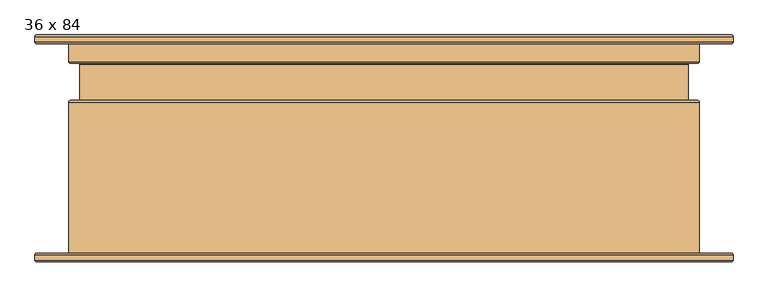
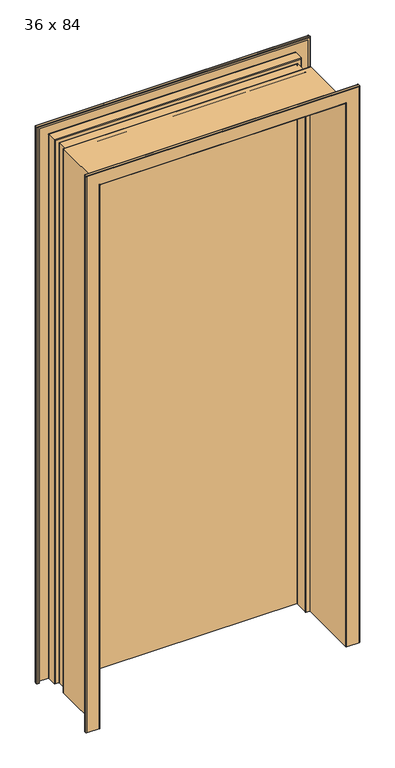
"""IFC4 building model written with IfcOpenShell, lengths in millimetres: door geometry, Door-Dunbarton_Doors-Hollow_Metal_Core : 36 x 84."""

from ifc_helpers import new_model, si_unit, frame, origin, origin_with_axes, place, context, project, spatial, polyline, circle_curve, ellipse_curve, outline, extrude, source, transform, mapped, element, save
from ifc_brep_helpers import plane_surface, cylinder_surface, revolved_surface, advanced_brep


def door_36_x_84_73b2aa22(model_context):
    return source(origin(), model_context, "Body", "SolidModel", [
        advanced_brep(
        [(-505.42825, -152.4635, 0.0), (-500.0625, -152.4635, 0.0), (-500.0625, -154.01925, 0.0), (-505.42825, -154.01925, 0.0), (-506.44425, -155.03525, 0.0), (-506.44425, -162.56, 0.0), (-505.42825, -163.576, 0.0), (-459.77175, -163.576, 0.0), (-458.75575, -162.56, 0.0), (-458.75575, 67.21475, 0.0), (-456.184, 69.7865, 0.0), (-443.89675, 69.7865, 0.0), (-442.88075, 70.8025, 0.0), (-442.88075, 122.5931, 0.0), (-443.89675, 123.6091, 0.0), (-456.184, 123.6091, 0.0), (-458.75575, 126.18085, 0.0), (-458.75575, 162.4965, 0.0), (-459.77175, 163.5125, 0.0), (-505.42825, 163.5125, 0.0), (-506.44425, 162.4965, 0.0), (-506.44425, 154.97175, 0.0), (-505.42825, 153.95575, 0.0), (-500.0625, 153.95575, 0.0), (-500.0625, 152.4, 0.0), (-505.42825, 152.4, 0.0), (-508.0, 154.97175, 0.0), (-508.0, 162.4965, 0.0), (-505.42825, 165.06825, 0.0), (-459.77175, 165.06825, 0.0), (-457.2, 162.4965, 0.0), (-457.2, 126.18085, 0.0), (-456.184, 125.16485, 0.0), (-443.89675, 125.16485, 0.0), (-441.325, 122.5931, 0.0), (-441.325, 70.8025, 0.0), (-443.89675, 68.23075, 0.0), (-456.184, 68.23075, 0.0), (-457.2, 67.21475, 0.0), (-457.2, -162.56, 0.0), (-459.77175, -165.13175, 0.0), (-505.42825, -165.13175, 0.0), (-508.0, -162.56, 0.0), (-508.0, -155.03525, 0.0), (-508.0, -155.03525, 2184.4), (-505.42825, -152.4635, 2181.82825), (-508.0, -162.56, 2184.4), (-505.42825, -165.13175, 2181.82825), (-459.77175, -165.13175, 2136.17175), (459.77175, -165.13175, 2136.17175), (459.77175, -165.13175, 0.0), (505.42825, -165.13175, 0.0), (505.42825, -165.13175, 2181.82825), (-457.2, -162.56, 2133.6), (-457.2, 67.21475, 2133.6), (-456.184, 68.23075, 2132.584), (-443.89675, 68.23075, 2120.29675), (443.89675, 68.23075, 2120.29675), (443.89675, 68.23075, 0.0), (456.184, 68.23075, 0.0), (456.184, 68.23075, 2132.584), (-441.325, 70.8025, 2117.725), (-441.325, 122.5931, 2117.725), (-443.89675, 125.16485, 2120.29675), (-456.184, 125.16485, 2132.584), (456.184, 125.16485, 2132.584), (456.184, 125.16485, 0.0), (443.89675, 125.16485, 0.0), (443.89675, 125.16485, 2120.29675), (-457.2, 126.18085, 2133.6), (-457.2, 162.4965, 2133.6), (-459.77175, 165.06825, 2136.17175), (-505.42825, 165.06825, 2181.82825), (505.42825, 165.06825, 2181.82825), (505.42825, 165.06825, 0.0), (459.77175, 165.06825, 0.0), (459.77175, 165.06825, 2136.17175), (-508.0, 162.4965, 2184.4), (-508.0, 154.97175, 2184.4), (-505.42825, 152.4, 2181.82825), (-500.0625, 152.4, 2176.4625), (500.0625, 152.4, 2176.4625), (500.0625, 152.4, 0.0), (505.42825, 152.4, 0.0), (505.42825, 152.4, 2181.82825), (-500.0625, 153.95575, 2176.4625), (-505.42825, 153.95575, 2181.82825), (505.42825, 153.95575, 2181.82825), (505.42825, 153.95575, 0.0), (500.0625, 153.95575, 0.0), (500.0625, 153.95575, 2176.4625), (-506.44425, 154.97175, 2182.84425), (-506.44425, 162.4965, 2182.84425), (-505.42825, 163.5125, 2181.82825), (-459.77175, 163.5125, 2136.17175), (459.77175, 163.5125, 2136.17175), (459.77175, 163.5125, 0.0), (505.42825, 163.5125, 0.0), (505.42825, 163.5125, 2181.82825), (-458.75575, 162.4965, 2135.15575), (-458.75575, 126.18085, 2135.15575), (-456.184, 123.6091, 2132.584), (-443.89675, 123.6091, 2120.29675), (443.89675, 123.6091, 2120.29675), (443.89675, 123.6091, 0.0), (456.184, 123.6091, 0.0), (456.184, 123.6091, 2132.584), (-442.88075, 122.5931, 2119.28075), (-442.88075, 70.8025, 2119.28075), (-443.89675, 69.7865, 2120.29675), (-456.184, 69.7865, 2132.584), (456.184, 69.7865, 2132.584), (456.184, 69.7865, 0.0), (443.89675, 69.7865, 0.0), (443.89675, 69.7865, 2120.29675), (-458.75575, 67.21475, 2135.15575), (-458.75575, -162.56, 2135.15575), (-459.77175, -163.576, 2136.17175), (-505.42825, -163.576, 2181.82825), (505.42825, -163.576, 2181.82825), (505.42825, -163.576, 0.0), (459.77175, -163.576, 0.0), (459.77175, -163.576, 2136.17175), (-506.44425, -162.56, 2182.84425), (-506.44425, -155.03525, 2182.84425), (-505.42825, -154.01925, 2181.82825), (-500.0625, -154.01925, 2176.4625), (500.0625, -154.01925, 2176.4625), (500.0625, -154.01925, 0.0), (505.42825, -154.01925, 0.0), (505.42825, -154.01925, 2181.82825), (-500.0625, -152.4635, 2176.4625), (505.42825, -152.4635, 2181.82825), (505.42825, -152.4635, 0.0), (500.0625, -152.4635, 0.0), (500.0625, -152.4635, 2176.4625), (508.0, -155.03525, 2184.4), (508.0, -162.56, 2184.4), (457.2, -162.56, 2133.6), (457.2, 67.21475, 2133.6), (441.325, 70.8025, 2117.725), (441.325, 122.5931, 2117.725), (457.2, 126.18085, 2133.6), (457.2, 162.4965, 2133.6), (508.0, 162.4965, 2184.4), (508.0, 154.97175, 2184.4), (506.44425, 154.97175, 2182.84425), (506.44425, 162.4965, 2182.84425), (458.75575, 162.4965, 2135.15575), (458.75575, 126.18085, 2135.15575), (442.88075, 122.5931, 2119.28075), (442.88075, 70.8025, 2119.28075), (458.75575, 67.21475, 2135.15575), (458.75575, -162.56, 2135.15575), (506.44425, -162.56, 2182.84425), (506.44425, -155.03525, 2182.84425), (508.0, -155.03525, 0.0), (508.0, -162.56, 0.0), (457.2, -162.56, 0.0), (457.2, 67.21475, 0.0), (441.325, 70.8025, 0.0), (441.325, 122.5931, 0.0), (457.2, 126.18085, 0.0), (457.2, 162.4965, 0.0), (508.0, 162.4965, 0.0), (508.0, 154.97175, 0.0), (506.44425, 154.97175, 0.0), (506.44425, 162.4965, 0.0), (458.75575, 162.4965, 0.0), (458.75575, 126.18085, 0.0), (442.88075, 122.5931, 0.0), (442.88075, 70.8025, 0.0), (458.75575, 67.21475, 0.0), (458.75575, -162.56, 0.0), (506.44425, -162.56, 0.0), (506.44425, -155.03525, 0.0)],
        [
            (0, 1),
            (1, 2),
            (2, 3),
            (3, 4, circle_curve(frame((-505.42825, -155.03525, 0.0), z_axis=(0.0, 0.0, 1.0), x_axis=(0.0, 1.0, 0.0)), 1.016)),
            (4, 5),
            (5, 6, circle_curve(frame((-505.42825, -162.56, 0.0), z_axis=(0.0, 0.0, 1.0), x_axis=(0.0, 1.0, 0.0)), 1.016)),
            (6, 7),
            (7, 8, circle_curve(frame((-459.77175, -162.56, 0.0), z_axis=(0.0, 0.0, 1.0), x_axis=(0.0, 1.0, 0.0)), 1.016)),
            (8, 9),
            (9, 10, circle_curve(frame((-456.184, 67.21475, 0.0), z_axis=(0.0, 0.0, -1.0), x_axis=(0.0, 1.0, 0.0)), 2.57175)),
            (10, 11),
            (11, 12, circle_curve(frame((-443.89675, 70.8025, 0.0), z_axis=(0.0, 0.0, 1.0), x_axis=(0.0, 1.0, 0.0)), 1.016)),
            (12, 13),
            (13, 14, circle_curve(frame((-443.89675, 122.5931, 0.0), z_axis=(0.0, 0.0, 1.0), x_axis=(0.0, 1.0, 0.0)), 1.016)),
            (14, 15),
            (15, 16, circle_curve(frame((-456.184, 126.18085, 0.0), z_axis=(0.0, 0.0, -1.0), x_axis=(0.0, 1.0, 0.0)), 2.57175)),
            (16, 17),
            (17, 18, circle_curve(frame((-459.77175, 162.4965, 0.0), z_axis=(0.0, 0.0, 1.0), x_axis=(0.0, 1.0, 0.0)), 1.016)),
            (18, 19),
            (19, 20, circle_curve(frame((-505.42825, 162.4965, 0.0), z_axis=(0.0, 0.0, 1.0), x_axis=(0.0, 1.0, 0.0)), 1.016)),
            (20, 21),
            (21, 22, circle_curve(frame((-505.42825, 154.97175, 0.0), z_axis=(0.0, 0.0, 1.0), x_axis=(0.0, 1.0, 0.0)), 1.016)),
            (22, 23),
            (23, 24),
            (24, 25),
            (25, 26, circle_curve(frame((-505.42825, 154.97175, 0.0), z_axis=(0.0, 0.0, -1.0), x_axis=(0.0, 1.0, 0.0)), 2.57175)),
            (26, 27),
            (27, 28, circle_curve(frame((-505.42825, 162.4965, 0.0), z_axis=(0.0, 0.0, -1.0), x_axis=(0.0, 1.0, 0.0)), 2.57175)),
            (28, 29),
            (29, 30, circle_curve(frame((-459.77175, 162.4965, 0.0), z_axis=(0.0, 0.0, -1.0), x_axis=(0.0, 1.0, 0.0)), 2.57175)),
            (30, 31),
            (31, 32, circle_curve(frame((-456.184, 126.18085, 0.0), z_axis=(0.0, 0.0, 1.0), x_axis=(0.0, 1.0, 0.0)), 1.016)),
            (32, 33),
            (33, 34, circle_curve(frame((-443.89675, 122.5931, 0.0), z_axis=(0.0, 0.0, -1.0), x_axis=(0.0, 1.0, 0.0)), 2.57175)),
            (34, 35),
            (35, 36, circle_curve(frame((-443.89675, 70.8025, 0.0), z_axis=(0.0, 0.0, -1.0), x_axis=(0.0, 1.0, 0.0)), 2.57175)),
            (36, 37),
            (37, 38, circle_curve(frame((-456.184, 67.21475, 0.0), z_axis=(0.0, 0.0, 1.0), x_axis=(0.0, 1.0, 0.0)), 1.016)),
            (38, 39),
            (39, 40, circle_curve(frame((-459.77175, -162.56, 0.0), z_axis=(0.0, 0.0, -1.0), x_axis=(0.0, 1.0, 0.0)), 2.57175)),
            (40, 41),
            (41, 42, circle_curve(frame((-505.42825, -162.56, 0.0), z_axis=(0.0, 0.0, -1.0), x_axis=(0.0, 1.0, 0.0)), 2.57175)),
            (42, 43),
            (43, 0, circle_curve(frame((-505.42825, -155.03525, 0.0), z_axis=(0.0, 0.0, -1.0), x_axis=(0.0, 1.0, 0.0)), 2.57175)),
            (43, 44),
            (44, 45, ellipse_curve(frame((-505.42825, -155.03525, 2181.82825), z_axis=(-0.7071067811865475, 0.0, -0.7071067811865475), x_axis=(0.7071067811865474, 0.0, -0.7071067811865476)), 3.6370037, 2.57175)),
            (45, 0),
            (42, 46),
            (46, 44),
            (41, 47),
            (47, 46, ellipse_curve(frame((-505.42825, -162.56, 2181.82825), z_axis=(-0.7071067811865475, 0.0, -0.7071067811865475), x_axis=(0.7071067811865474, 0.0, -0.7071067811865476)), 3.6370037, 2.57175)),
            (40, 48),
            (48, 49),
            (49, 50),
            (50, 51),
            (51, 52),
            (52, 47),
            (39, 53),
            (53, 48, ellipse_curve(frame((-459.77175, -162.56, 2136.17175), z_axis=(-0.7071067811865475, 0.0, -0.7071067811865475), x_axis=(0.7071067811865474, 0.0, -0.7071067811865476)), 3.6370037, 2.57175)),
            (38, 54),
            (54, 53),
            (37, 55),
            (55, 54, ellipse_curve(frame((-456.184, 67.21475, 2132.584), z_axis=(0.7071067811865475, 0.0, 0.7071067811865475), x_axis=(-0.7071067811865474, 0.0, 0.7071067811865476)), 1.436841, 1.016)),
            (36, 56),
            (56, 57),
            (57, 58),
            (58, 59),
            (59, 60),
            (60, 55),
            (35, 61),
            (61, 56, ellipse_curve(frame((-443.89675, 70.8025, 2120.29675), z_axis=(-0.7071067811865475, 0.0, -0.7071067811865475), x_axis=(0.7071067811865474, 0.0, -0.7071067811865476)), 3.6370037, 2.57175)),
            (34, 62),
            (62, 61),
            (33, 63),
            (63, 62, ellipse_curve(frame((-443.89675, 122.5931, 2120.29675), z_axis=(-0.7071067811865475, 0.0, -0.7071067811865475), x_axis=(0.7071067811865474, 0.0, -0.7071067811865476)), 3.6370037, 2.57175)),
            (32, 64),
            (64, 65),
            (65, 66),
            (66, 67),
            (67, 68),
            (68, 63),
            (31, 69),
            (69, 64, ellipse_curve(frame((-456.184, 126.18085, 2132.584), z_axis=(0.7071067811865475, 0.0, 0.7071067811865475), x_axis=(-0.7071067811865474, 0.0, 0.7071067811865476)), 1.436841, 1.016)),
            (30, 70),
            (70, 69),
            (29, 71),
            (71, 70, ellipse_curve(frame((-459.77175, 162.4965, 2136.17175), z_axis=(-0.7071067811865475, 0.0, -0.7071067811865475), x_axis=(0.7071067811865474, 0.0, -0.7071067811865476)), 3.6370037, 2.57175)),
            (28, 72),
            (72, 73),
            (73, 74),
            (74, 75),
            (75, 76),
            (76, 71),
            (27, 77),
            (77, 72, ellipse_curve(frame((-505.42825, 162.4965, 2181.82825), z_axis=(-0.7071067811865475, 0.0, -0.7071067811865475), x_axis=(0.7071067811865474, 0.0, -0.7071067811865476)), 3.6370037, 2.57175)),
            (26, 78),
            (78, 77),
            (25, 79),
            (79, 78, ellipse_curve(frame((-505.42825, 154.97175, 2181.82825), z_axis=(-0.7071067811865475, 0.0, -0.7071067811865475), x_axis=(0.7071067811865474, 0.0, -0.7071067811865476)), 3.6370037, 2.57175)),
            (24, 80),
            (80, 81),
            (81, 82),
            (82, 83),
            (83, 84),
            (84, 79),
            (23, 85),
            (85, 80),
            (22, 86),
            (86, 87),
            (87, 88),
            (88, 89),
            (89, 90),
            (90, 85),
            (21, 91),
            (91, 86, ellipse_curve(frame((-505.42825, 154.97175, 2181.82825), z_axis=(0.7071067811865475, 0.0, 0.7071067811865475), x_axis=(-0.7071067811865474, 0.0, 0.7071067811865476)), 1.436841, 1.016)),
            (20, 92),
            (92, 91),
            (19, 93),
            (93, 92, ellipse_curve(frame((-505.42825, 162.4965, 2181.82825), z_axis=(0.7071067811865475, 0.0, 0.7071067811865475), x_axis=(-0.7071067811865474, 0.0, 0.7071067811865476)), 1.436841, 1.016)),
            (18, 94),
            (94, 95),
            (95, 96),
            (96, 97),
            (97, 98),
            (98, 93),
            (17, 99),
            (99, 94, ellipse_curve(frame((-459.77175, 162.4965, 2136.17175), z_axis=(0.7071067811865475, 0.0, 0.7071067811865475), x_axis=(-0.7071067811865474, 0.0, 0.7071067811865476)), 1.436841, 1.016)),
            (16, 100),
            (100, 99),
            (15, 101),
            (101, 100, ellipse_curve(frame((-456.184, 126.18085, 2132.584), z_axis=(-0.7071067811865475, 0.0, -0.7071067811865475), x_axis=(0.7071067811865474, 0.0, -0.7071067811865476)), 3.6370037, 2.57175)),
            (14, 102),
            (102, 103),
            (103, 104),
            (104, 105),
            (105, 106),
            (106, 101),
            (13, 107),
            (107, 102, ellipse_curve(frame((-443.89675, 122.5931, 2120.29675), z_axis=(0.7071067811865475, 0.0, 0.7071067811865475), x_axis=(-0.7071067811865474, 0.0, 0.7071067811865476)), 1.436841, 1.016)),
            (12, 108),
            (108, 107),
            (11, 109),
            (109, 108, ellipse_curve(frame((-443.89675, 70.8025, 2120.29675), z_axis=(0.7071067811865475, 0.0, 0.7071067811865475), x_axis=(-0.7071067811865474, 0.0, 0.7071067811865476)), 1.436841, 1.016)),
            (10, 110),
            (110, 111),
            (111, 112),
            (112, 113),
            (113, 114),
            (114, 109),
            (9, 115),
            (115, 110, ellipse_curve(frame((-456.184, 67.21475, 2132.584), z_axis=(-0.7071067811865475, 0.0, -0.7071067811865475), x_axis=(0.7071067811865474, 0.0, -0.7071067811865476)), 3.6370037, 2.57175)),
            (8, 116),
            (116, 115),
            (7, 117),
            (117, 116, ellipse_curve(frame((-459.77175, -162.56, 2136.17175), z_axis=(0.7071067811865475, 0.0, 0.7071067811865475), x_axis=(-0.7071067811865474, 0.0, 0.7071067811865476)), 1.436841, 1.016)),
            (6, 118),
            (118, 119),
            (119, 120),
            (120, 121),
            (121, 122),
            (122, 117),
            (5, 123),
            (123, 118, ellipse_curve(frame((-505.42825, -162.56, 2181.82825), z_axis=(0.7071067811865475, 0.0, 0.7071067811865475), x_axis=(-0.7071067811865474, 0.0, 0.7071067811865476)), 1.436841, 1.016)),
            (4, 124),
            (124, 123),
            (3, 125),
            (125, 124, ellipse_curve(frame((-505.42825, -155.03525, 2181.82825), z_axis=(0.7071067811865475, 0.0, 0.7071067811865475), x_axis=(-0.7071067811865474, 0.0, 0.7071067811865476)), 1.436841, 1.016)),
            (2, 126),
            (126, 127),
            (127, 128),
            (128, 129),
            (129, 130),
            (130, 125),
            (1, 131),
            (131, 126),
            (45, 132),
            (132, 133),
            (133, 134),
            (134, 135),
            (135, 131),
            (44, 136),
            (136, 132, ellipse_curve(frame((505.42825, -155.03525, 2181.82825), z_axis=(-0.7071067811865475, 0.0, 0.7071067811865475), x_axis=(-0.7071067811865476, 0.0, -0.7071067811865474)), 3.6370037, 2.57175)),
            (46, 137),
            (137, 136),
            (52, 137, ellipse_curve(frame((505.42825, -162.56, 2181.82825), z_axis=(-0.7071067811865475, 0.0, 0.7071067811865475), x_axis=(-0.7071067811865476, 0.0, -0.7071067811865474)), 3.6370037, 2.57175)),
            (53, 138),
            (138, 49, ellipse_curve(frame((459.77175, -162.56, 2136.17175), z_axis=(-0.7071067811865475, 0.0, 0.7071067811865475), x_axis=(-0.7071067811865476, 0.0, -0.7071067811865474)), 3.6370037, 2.57175)),
            (54, 139),
            (139, 138),
            (60, 139, ellipse_curve(frame((456.184, 67.21475, 2132.584), z_axis=(0.7071067811865475, 0.0, -0.7071067811865475), x_axis=(0.7071067811865476, 0.0, 0.7071067811865474)), 1.436841, 1.016)),
            (61, 140),
            (140, 57, ellipse_curve(frame((443.89675, 70.8025, 2120.29675), z_axis=(-0.7071067811865475, 0.0, 0.7071067811865475), x_axis=(-0.7071067811865476, 0.0, -0.7071067811865474)), 3.6370037, 2.57175)),
            (62, 141),
            (141, 140),
            (68, 141, ellipse_curve(frame((443.89675, 122.5931, 2120.29675), z_axis=(-0.7071067811865475, 0.0, 0.7071067811865475), x_axis=(-0.7071067811865476, 0.0, -0.7071067811865474)), 3.6370037, 2.57175)),
            (69, 142),
            (142, 65, ellipse_curve(frame((456.184, 126.18085, 2132.584), z_axis=(0.7071067811865475, 0.0, -0.7071067811865475), x_axis=(0.7071067811865476, 0.0, 0.7071067811865474)), 1.436841, 1.016)),
            (70, 143),
            (143, 142),
            (76, 143, ellipse_curve(frame((459.77175, 162.4965, 2136.17175), z_axis=(-0.7071067811865475, 0.0, 0.7071067811865475), x_axis=(-0.7071067811865476, 0.0, -0.7071067811865474)), 3.6370037, 2.57175)),
            (77, 144),
            (144, 73, ellipse_curve(frame((505.42825, 162.4965, 2181.82825), z_axis=(-0.7071067811865475, 0.0, 0.7071067811865475), x_axis=(-0.7071067811865476, 0.0, -0.7071067811865474)), 3.6370037, 2.57175)),
            (78, 145),
            (145, 144),
            (84, 145, ellipse_curve(frame((505.42825, 154.97175, 2181.82825), z_axis=(-0.7071067811865475, 0.0, 0.7071067811865475), x_axis=(-0.7071067811865476, 0.0, -0.7071067811865474)), 3.6370037, 2.57175)),
            (90, 81),
            (91, 146),
            (146, 87, ellipse_curve(frame((505.42825, 154.97175, 2181.82825), z_axis=(0.7071067811865475, 0.0, -0.7071067811865475), x_axis=(0.7071067811865476, 0.0, 0.7071067811865474)), 1.436841, 1.016)),
            (92, 147),
            (147, 146),
            (98, 147, ellipse_curve(frame((505.42825, 162.4965, 2181.82825), z_axis=(0.7071067811865475, 0.0, -0.7071067811865475), x_axis=(0.7071067811865476, 0.0, 0.7071067811865474)), 1.436841, 1.016)),
            (99, 148),
            (148, 95, ellipse_curve(frame((459.77175, 162.4965, 2136.17175), z_axis=(0.7071067811865475, 0.0, -0.7071067811865475), x_axis=(0.7071067811865476, 0.0, 0.7071067811865474)), 1.436841, 1.016)),
            (100, 149),
            (149, 148),
            (106, 149, ellipse_curve(frame((456.184, 126.18085, 2132.584), z_axis=(-0.7071067811865475, 0.0, 0.7071067811865475), x_axis=(-0.7071067811865476, 0.0, -0.7071067811865474)), 3.6370037, 2.57175)),
            (107, 150),
            (150, 103, ellipse_curve(frame((443.89675, 122.5931, 2120.29675), z_axis=(0.7071067811865475, 0.0, -0.7071067811865475), x_axis=(0.7071067811865476, 0.0, 0.7071067811865474)), 1.436841, 1.016)),
            (108, 151),
            (151, 150),
            (114, 151, ellipse_curve(frame((443.89675, 70.8025, 2120.29675), z_axis=(0.7071067811865475, 0.0, -0.7071067811865475), x_axis=(0.7071067811865476, 0.0, 0.7071067811865474)), 1.436841, 1.016)),
            (115, 152),
            (152, 111, ellipse_curve(frame((456.184, 67.21475, 2132.584), z_axis=(-0.7071067811865475, 0.0, 0.7071067811865475), x_axis=(-0.7071067811865476, 0.0, -0.7071067811865474)), 3.6370037, 2.57175)),
            (116, 153),
            (153, 152),
            (122, 153, ellipse_curve(frame((459.77175, -162.56, 2136.17175), z_axis=(0.7071067811865475, 0.0, -0.7071067811865475), x_axis=(0.7071067811865476, 0.0, 0.7071067811865474)), 1.436841, 1.016)),
            (123, 154),
            (154, 119, ellipse_curve(frame((505.42825, -162.56, 2181.82825), z_axis=(0.7071067811865475, 0.0, -0.7071067811865475), x_axis=(0.7071067811865476, 0.0, 0.7071067811865474)), 1.436841, 1.016)),
            (124, 155),
            (155, 154),
            (130, 155, ellipse_curve(frame((505.42825, -155.03525, 2181.82825), z_axis=(0.7071067811865475, 0.0, -0.7071067811865475), x_axis=(0.7071067811865476, 0.0, 0.7071067811865474)), 1.436841, 1.016)),
            (135, 127),
            (133, 156, circle_curve(frame((505.42825, -155.03525, 0.0), z_axis=(0.0, 0.0, -1.0), x_axis=(0.0, 1.0, 0.0)), 2.57175)),
            (156, 157),
            (157, 51, circle_curve(frame((505.42825, -162.56, 0.0), z_axis=(0.0, 0.0, -1.0), x_axis=(0.0, 1.0, 0.0)), 2.57175)),
            (50, 158, circle_curve(frame((459.77175, -162.56, 0.0), z_axis=(0.0, 0.0, -1.0), x_axis=(0.0, 1.0, 0.0)), 2.57175)),
            (158, 159),
            (159, 59, circle_curve(frame((456.184, 67.21475, 0.0), z_axis=(0.0, 0.0, 1.0), x_axis=(0.0, 1.0, 0.0)), 1.016)),
            (58, 160, circle_curve(frame((443.89675, 70.8025, 0.0), z_axis=(0.0, 0.0, -1.0), x_axis=(0.0, 1.0, 0.0)), 2.57175)),
            (160, 161),
            (161, 67, circle_curve(frame((443.89675, 122.5931, 0.0), z_axis=(0.0, 0.0, -1.0), x_axis=(0.0, 1.0, 0.0)), 2.57175)),
            (66, 162, circle_curve(frame((456.184, 126.18085, 0.0), z_axis=(0.0, 0.0, 1.0), x_axis=(0.0, 1.0, 0.0)), 1.016)),
            (162, 163),
            (163, 75, circle_curve(frame((459.77175, 162.4965, 0.0), z_axis=(0.0, 0.0, -1.0), x_axis=(0.0, 1.0, 0.0)), 2.57175)),
            (74, 164, circle_curve(frame((505.42825, 162.4965, 0.0), z_axis=(0.0, 0.0, -1.0), x_axis=(0.0, 1.0, 0.0)), 2.57175)),
            (164, 165),
            (165, 83, circle_curve(frame((505.42825, 154.97175, 0.0), z_axis=(0.0, 0.0, -1.0), x_axis=(0.0, 1.0, 0.0)), 2.57175)),
            (82, 89),
            (88, 166, circle_curve(frame((505.42825, 154.97175, 0.0), z_axis=(0.0, 0.0, 1.0), x_axis=(0.0, 1.0, 0.0)), 1.016)),
            (166, 167),
            (167, 97, circle_curve(frame((505.42825, 162.4965, 0.0), z_axis=(0.0, 0.0, 1.0), x_axis=(0.0, 1.0, 0.0)), 1.016)),
            (96, 168, circle_curve(frame((459.77175, 162.4965, 0.0), z_axis=(0.0, 0.0, 1.0), x_axis=(0.0, 1.0, 0.0)), 1.016)),
            (168, 169),
            (169, 105, circle_curve(frame((456.184, 126.18085, 0.0), z_axis=(0.0, 0.0, -1.0), x_axis=(0.0, 1.0, 0.0)), 2.57175)),
            (104, 170, circle_curve(frame((443.89675, 122.5931, 0.0), z_axis=(0.0, 0.0, 1.0), x_axis=(0.0, 1.0, 0.0)), 1.016)),
            (170, 171),
            (171, 113, circle_curve(frame((443.89675, 70.8025, 0.0), z_axis=(0.0, 0.0, 1.0), x_axis=(0.0, 1.0, 0.0)), 1.016)),
            (112, 172, circle_curve(frame((456.184, 67.21475, 0.0), z_axis=(0.0, 0.0, -1.0), x_axis=(0.0, 1.0, 0.0)), 2.57175)),
            (172, 173),
            (173, 121, circle_curve(frame((459.77175, -162.56, 0.0), z_axis=(0.0, 0.0, 1.0), x_axis=(0.0, 1.0, 0.0)), 1.016)),
            (120, 174, circle_curve(frame((505.42825, -162.56, 0.0), z_axis=(0.0, 0.0, 1.0), x_axis=(0.0, 1.0, 0.0)), 1.016)),
            (174, 175),
            (175, 129, circle_curve(frame((505.42825, -155.03525, 0.0), z_axis=(0.0, 0.0, 1.0), x_axis=(0.0, 1.0, 0.0)), 1.016)),
            (128, 134),
            (136, 156),
            (137, 157),
            (138, 158),
            (139, 159),
            (140, 160),
            (141, 161),
            (142, 162),
            (143, 163),
            (144, 164),
            (145, 165),
            (146, 166),
            (147, 167),
            (148, 168),
            (149, 169),
            (150, 170),
            (151, 171),
            (152, 172),
            (153, 173),
            (154, 174),
            (155, 175),
        ],
        [
            plane_surface(frame((-468.3125, 152.4, 0.0), z_axis=(0.0, 0.0, -1.0), x_axis=(1.0, 0.0, 0.0))),
            cylinder_surface(frame((-505.42825, -155.03525, 0.0), z_axis=(0.0, 0.0, -1.0), x_axis=(0.0, 1.0, 0.0)), 2.57175),
            plane_surface(frame((-508.0, -155.03525, 0.0), z_axis=(-1.0, 0.0, 0.0), x_axis=(0.0, 0.0, 1.0))),
            cylinder_surface(frame((-505.42825, -162.56, 0.0), z_axis=(0.0, 0.0, -1.0), x_axis=(0.0, 1.0, 0.0)), 2.57175),
            plane_surface(frame((-505.42825, -165.13175, 0.0), z_axis=(0.0, -1.0, 0.0), x_axis=(0.0, 0.0, 1.0))),
            cylinder_surface(frame((-459.77175, -162.56, 0.0), z_axis=(0.0, 0.0, -1.0), x_axis=(0.0, 1.0, 0.0)), 2.57175),
            plane_surface(frame((-457.2, -162.56, 0.0), z_axis=(1.0, 0.0, 0.0), x_axis=(0.0, 0.0, 1.0))),
            revolved_surface(polyline([(-456.184, 68.23075, 2133.600000014587), (-456.184, 68.23075, 0.0)]), (-456.184, 67.21475, 0.0), (0.0, 0.0, 1.0)),
            plane_surface(frame((-456.184, 68.23075, 0.0), z_axis=(0.0, -1.0, 0.0), x_axis=(0.0, 0.0, 1.0))),
            cylinder_surface(frame((-443.89675, 70.8025, 0.0), z_axis=(0.0, 0.0, -1.0), x_axis=(0.0, 1.0, 0.0)), 2.57175),
            plane_surface(frame((-441.325, 70.8025, 0.0), z_axis=(1.0, 0.0, 0.0), x_axis=(0.0, 0.0, 1.0))),
            cylinder_surface(frame((-443.89675, 122.5931, 0.0), z_axis=(0.0, 0.0, -1.0), x_axis=(0.0, 1.0, 0.0)), 2.57175),
            plane_surface(frame((-443.89675, 125.16485, 0.0), z_axis=(0.0, 1.0, 0.0), x_axis=(0.0, 0.0, 1.0))),
            revolved_surface(polyline([(-456.184, 127.19685000000001, 2133.600000014587), (-456.184, 127.19685000000001, 0.0)]), (-456.184, 126.18085, 0.0), (0.0, 0.0, 1.0)),
            plane_surface(frame((-457.2, 126.18085, 0.0), z_axis=(1.0, 0.0, 0.0), x_axis=(0.0, 0.0, 1.0))),
            cylinder_surface(frame((-459.77175, 162.4965, 0.0), z_axis=(0.0, 0.0, -1.0), x_axis=(0.0, 1.0, 0.0)), 2.57175),
            plane_surface(frame((-459.77175, 165.06825, 0.0), z_axis=(0.0, 1.0, 0.0), x_axis=(0.0, 0.0, 1.0))),
            cylinder_surface(frame((-505.42825, 162.4965, 0.0), z_axis=(0.0, 0.0, -1.0), x_axis=(0.0, 1.0, 0.0)), 2.57175),
            plane_surface(frame((-508.0, 162.4965, 0.0), z_axis=(-1.0, 0.0, 0.0), x_axis=(0.0, 0.0, 1.0))),
            cylinder_surface(frame((-505.42825, 154.97175, 0.0), z_axis=(0.0, 0.0, -1.0), x_axis=(0.0, 1.0, 0.0)), 2.57175),
            plane_surface(frame((-505.42825, 152.4, 0.0), z_axis=(0.0, -1.0, 0.0), x_axis=(0.0, 0.0, 1.0))),
            plane_surface(frame((-500.0625, 152.4, 0.0), z_axis=(1.0, 0.0, 0.0), x_axis=(0.0, 0.0, 1.0))),
            plane_surface(frame((-500.0625, 153.95575, 0.0), z_axis=(0.0, 1.0, 0.0), x_axis=(0.0, 0.0, 1.0))),
            revolved_surface(polyline([(-505.42825, 155.98774999999998, 2182.844250014587), (-505.42825, 155.98774999999998, 0.0)]), (-505.42825, 154.97175, 0.0), (0.0, 0.0, 1.0)),
            plane_surface(frame((-506.44425, 154.97175, 0.0), z_axis=(1.0, 0.0, 0.0), x_axis=(0.0, 0.0, 1.0))),
            revolved_surface(polyline([(-505.42825, 163.5125, 2182.844250014587), (-505.42825, 163.5125, 0.0)]), (-505.42825, 162.4965, 0.0), (0.0, 0.0, 1.0)),
            plane_surface(frame((-505.42825, 163.5125, 0.0), z_axis=(0.0, -1.0, 0.0), x_axis=(0.0, 0.0, 1.0))),
            revolved_surface(polyline([(-459.77175, 163.5125, 2137.187750014587), (-459.77175, 163.5125, 0.0)]), (-459.77175, 162.4965, 0.0), (0.0, 0.0, 1.0)),
            plane_surface(frame((-458.75575, 162.4965, 0.0), z_axis=(-1.0, 0.0, 0.0), x_axis=(0.0, 0.0, 1.0))),
            cylinder_surface(frame((-456.184, 126.18085, 0.0), z_axis=(0.0, 0.0, -1.0), x_axis=(0.0, 1.0, 0.0)), 2.57175),
            plane_surface(frame((-456.184, 123.6091, 0.0), z_axis=(0.0, -1.0, 0.0), x_axis=(0.0, 0.0, 1.0))),
            revolved_surface(polyline([(-443.89675, 123.60910000000001, 2121.312750014587), (-443.89675, 123.60910000000001, 0.0)]), (-443.89675, 122.5931, 0.0), (0.0, 0.0, 1.0)),
            plane_surface(frame((-442.88075, 122.5931, 0.0), z_axis=(-1.0, 0.0, 0.0), x_axis=(0.0, 0.0, 1.0))),
            revolved_surface(polyline([(-443.89675, 71.8185, 2121.312750014587), (-443.89675, 71.8185, 0.0)]), (-443.89675, 70.8025, 0.0), (0.0, 0.0, 1.0)),
            plane_surface(frame((-443.89675, 69.7865, 0.0), z_axis=(0.0, 1.0, 0.0), x_axis=(0.0, 0.0, 1.0))),
            cylinder_surface(frame((-456.184, 67.21475, 0.0), z_axis=(0.0, 0.0, -1.0), x_axis=(0.0, 1.0, 0.0)), 2.57175),
            plane_surface(frame((-458.75575, 67.21475, 0.0), z_axis=(-1.0, 0.0, 0.0), x_axis=(0.0, 0.0, 1.0))),
            revolved_surface(polyline([(-459.77175, -161.544, 2137.187750014587), (-459.77175, -161.544, 0.0)]), (-459.77175, -162.56, 0.0), (0.0, 0.0, 1.0)),
            plane_surface(frame((-459.77175, -163.576, 0.0), z_axis=(0.0, 1.0, 0.0), x_axis=(0.0, 0.0, 1.0))),
            revolved_surface(polyline([(-505.42825, -161.544, 2182.844250014587), (-505.42825, -161.544, 0.0)]), (-505.42825, -162.56, 0.0), (0.0, 0.0, 1.0)),
            plane_surface(frame((-506.44425, -162.56, 0.0), z_axis=(1.0, 0.0, 0.0), x_axis=(0.0, 0.0, 1.0))),
            revolved_surface(polyline([(-505.42825, -154.01925, 2182.844250014587), (-505.42825, -154.01925, 0.0)]), (-505.42825, -155.03525, 0.0), (0.0, 0.0, 1.0)),
            plane_surface(frame((-505.42825, -154.01925, 0.0), z_axis=(0.0, -1.0, 0.0), x_axis=(0.0, 0.0, 1.0))),
            plane_surface(frame((-500.0625, -154.01925, 0.0), z_axis=(1.0, 0.0, 0.0), x_axis=(0.0, 0.0, 1.0))),
            plane_surface(frame((-500.0625, -152.4635, 0.0), z_axis=(0.0, 1.0, 0.0), x_axis=(0.0, 0.0, 1.0))),
            cylinder_surface(frame((-468.3125, -155.03525, 2181.82825), z_axis=(-1.0, 0.0, 0.0), x_axis=(0.0, 1.0, 0.0)), 2.57175),
            plane_surface(frame((-508.0, -155.03525, 2184.4), z_axis=(0.0, 0.0, 1.0), x_axis=(1.0, 0.0, 0.0))),
            cylinder_surface(frame((-468.3125, -162.56, 2181.82825), z_axis=(-1.0, 0.0, 0.0), x_axis=(0.0, 1.0, 0.0)), 2.57175),
            cylinder_surface(frame((-468.3125, -162.56, 2136.17175), z_axis=(-1.0, 0.0, 0.0), x_axis=(0.0, 1.0, 0.0)), 2.57175),
            plane_surface(frame((-457.2, -162.56, 2133.6), z_axis=(0.0, 0.0, -1.0), x_axis=(1.0, 0.0, 0.0))),
            revolved_surface(polyline([(457.20000001458686, 68.23075, 2132.584), (-457.20000001458686, 68.23075, 2132.584)]), (-468.3125, 67.21475, 2132.584), (1.0, 0.0, 0.0)),
            cylinder_surface(frame((-468.3125, 70.8025, 2120.29675), z_axis=(-1.0, 0.0, 0.0), x_axis=(0.0, 1.0, 0.0)), 2.57175),
            plane_surface(frame((-441.325, 70.8025, 2117.725), z_axis=(0.0, 0.0, -1.0), x_axis=(1.0, 0.0, 0.0))),
            cylinder_surface(frame((-468.3125, 122.5931, 2120.29675), z_axis=(-1.0, 0.0, 0.0), x_axis=(0.0, 1.0, 0.0)), 2.57175),
            revolved_surface(polyline([(457.20000001458686, 127.19685000000001, 2132.584), (-457.20000001458686, 127.19685000000001, 2132.584)]), (-468.3125, 126.18085, 2132.584), (1.0, 0.0, 0.0)),
            plane_surface(frame((-457.2, 126.18085, 2133.6), z_axis=(0.0, 0.0, -1.0), x_axis=(1.0, 0.0, 0.0))),
            cylinder_surface(frame((-468.3125, 162.4965, 2136.17175), z_axis=(-1.0, 0.0, 0.0), x_axis=(0.0, 1.0, 0.0)), 2.57175),
            cylinder_surface(frame((-468.3125, 162.4965, 2181.82825), z_axis=(-1.0, 0.0, 0.0), x_axis=(0.0, 1.0, 0.0)), 2.57175),
            plane_surface(frame((-508.0, 162.4965, 2184.4), z_axis=(0.0, 0.0, 1.0), x_axis=(1.0, 0.0, 0.0))),
            cylinder_surface(frame((-468.3125, 154.97175, 2181.82825), z_axis=(-1.0, 0.0, 0.0), x_axis=(0.0, 1.0, 0.0)), 2.57175),
            plane_surface(frame((-500.0625, 152.4, 2176.4625), z_axis=(0.0, 0.0, -1.0), x_axis=(1.0, 0.0, 0.0))),
            revolved_surface(polyline([(506.4442500145868, 155.98774999999998, 2181.82825), (-506.4442500145868, 155.98774999999998, 2181.82825)]), (-468.3125, 154.97175, 2181.82825), (1.0, 0.0, 0.0)),
            plane_surface(frame((-506.44425, 154.97175, 2182.84425), z_axis=(0.0, 0.0, -1.0), x_axis=(1.0, 0.0, 0.0))),
            revolved_surface(polyline([(506.4442500145868, 163.5125, 2181.82825), (-506.4442500145868, 163.5125, 2181.82825)]), (-468.3125, 162.4965, 2181.82825), (1.0, 0.0, 0.0)),
            revolved_surface(polyline([(460.7877500145869, 163.5125, 2136.17175), (-460.78775001458683, 163.5125, 2136.17175)]), (-468.3125, 162.4965, 2136.17175), (1.0, 0.0, 0.0)),
            plane_surface(frame((-458.75575, 162.4965, 2135.15575), z_axis=(0.0, 0.0, 1.0), x_axis=(1.0, 0.0, 0.0))),
            cylinder_surface(frame((-468.3125, 126.18085, 2132.584), z_axis=(-1.0, 0.0, 0.0), x_axis=(0.0, 1.0, 0.0)), 2.57175),
            revolved_surface(polyline([(444.9127500145869, 123.60910000000001, 2120.29675), (-444.91275001458683, 123.60910000000001, 2120.29675)]), (-468.3125, 122.5931, 2120.29675), (1.0, 0.0, 0.0)),
            plane_surface(frame((-442.88075, 122.5931, 2119.28075), z_axis=(0.0, 0.0, 1.0), x_axis=(1.0, 0.0, 0.0))),
            revolved_surface(polyline([(444.9127500145869, 71.8185, 2120.29675), (-444.91275001458683, 71.8185, 2120.29675)]), (-468.3125, 70.8025, 2120.29675), (1.0, 0.0, 0.0)),
            cylinder_surface(frame((-468.3125, 67.21475, 2132.584), z_axis=(-1.0, 0.0, 0.0), x_axis=(0.0, 1.0, 0.0)), 2.57175),
            plane_surface(frame((-458.75575, 67.21475, 2135.15575), z_axis=(0.0, 0.0, 1.0), x_axis=(1.0, 0.0, 0.0))),
            revolved_surface(polyline([(460.7877500145869, -161.544, 2136.17175), (-460.78775001458683, -161.544, 2136.17175)]), (-468.3125, -162.56, 2136.17175), (1.0, 0.0, 0.0)),
            revolved_surface(polyline([(506.4442500145868, -161.544, 2181.82825), (-506.4442500145868, -161.544, 2181.82825)]), (-468.3125, -162.56, 2181.82825), (1.0, 0.0, 0.0)),
            plane_surface(frame((-506.44425, -162.56, 2182.84425), z_axis=(0.0, 0.0, -1.0), x_axis=(1.0, 0.0, 0.0))),
            revolved_surface(polyline([(506.4442500145868, -154.01925, 2181.82825), (-506.4442500145868, -154.01925, 2181.82825)]), (-468.3125, -155.03525, 2181.82825), (1.0, 0.0, 0.0)),
            plane_surface(frame((-500.0625, -154.01925, 2176.4625), z_axis=(0.0, 0.0, -1.0), x_axis=(1.0, 0.0, 0.0))),
            plane_surface(frame((468.3125, 152.4, 0.0), z_axis=(0.0, 0.0, -1.0), x_axis=(-1.0, 0.0, 0.0))),
            cylinder_surface(frame((505.42825, -155.03525, 2144.7125), z_axis=(0.0, 0.0, 1.0), x_axis=(0.0, 1.0, 0.0)), 2.57175),
            plane_surface(frame((508.0, -155.03525, 2184.4), z_axis=(1.0, 0.0, 0.0), x_axis=(0.0, 0.0, -1.0))),
            cylinder_surface(frame((505.42825, -162.56, 2144.7125), z_axis=(0.0, 0.0, 1.0), x_axis=(0.0, 1.0, 0.0)), 2.57175),
            cylinder_surface(frame((459.77175, -162.56, 2144.7125), z_axis=(0.0, 0.0, 1.0), x_axis=(0.0, 1.0, 0.0)), 2.57175),
            plane_surface(frame((457.2, -162.56, 2133.6), z_axis=(-1.0, 0.0, 0.0), x_axis=(0.0, 0.0, -1.0))),
            revolved_surface(polyline([(456.184, 68.23075, 0.0), (456.184, 68.23075, 2133.600000014587)]), (456.184, 67.21475, 2144.7125), (0.0, 0.0, -1.0)),
            cylinder_surface(frame((443.89675, 70.8025, 2144.7125), z_axis=(0.0, 0.0, 1.0), x_axis=(0.0, 1.0, 0.0)), 2.57175),
            plane_surface(frame((441.325, 70.8025, 2117.725), z_axis=(-1.0, 0.0, 0.0), x_axis=(0.0, 0.0, -1.0))),
            cylinder_surface(frame((443.89675, 122.5931, 2144.7125), z_axis=(0.0, 0.0, 1.0), x_axis=(0.0, 1.0, 0.0)), 2.57175),
            revolved_surface(polyline([(456.184, 127.19685000000001, 0.0), (456.184, 127.19685000000001, 2133.600000014587)]), (456.184, 126.18085, 2144.7125), (0.0, 0.0, -1.0)),
            plane_surface(frame((457.2, 126.18085, 2133.6), z_axis=(-1.0, 0.0, 0.0), x_axis=(0.0, 0.0, -1.0))),
            cylinder_surface(frame((459.77175, 162.4965, 2144.7125), z_axis=(0.0, 0.0, 1.0), x_axis=(0.0, 1.0, 0.0)), 2.57175),
            cylinder_surface(frame((505.42825, 162.4965, 2144.7125), z_axis=(0.0, 0.0, 1.0), x_axis=(0.0, 1.0, 0.0)), 2.57175),
            plane_surface(frame((508.0, 162.4965, 2184.4), z_axis=(1.0, 0.0, 0.0), x_axis=(0.0, 0.0, -1.0))),
            cylinder_surface(frame((505.42825, 154.97175, 2144.7125), z_axis=(0.0, 0.0, 1.0), x_axis=(0.0, 1.0, 0.0)), 2.57175),
            plane_surface(frame((500.0625, 152.4, 2176.4625), z_axis=(-1.0, 0.0, 0.0), x_axis=(0.0, 0.0, -1.0))),
            revolved_surface(polyline([(505.42825, 155.98774999999998, 0.0), (505.42825, 155.98774999999998, 2182.844250014587)]), (505.42825, 154.97175, 2144.7125), (0.0, 0.0, -1.0)),
            plane_surface(frame((506.44425, 154.97175, 2182.84425), z_axis=(-1.0, 0.0, 0.0), x_axis=(0.0, 0.0, -1.0))),
            revolved_surface(polyline([(505.42825, 163.5125, 0.0), (505.42825, 163.5125, 2182.844250014587)]), (505.42825, 162.4965, 2144.7125), (0.0, 0.0, -1.0)),
            revolved_surface(polyline([(459.77175, 163.5125, 0.0), (459.77175, 163.5125, 2137.187750014587)]), (459.77175, 162.4965, 2144.7125), (0.0, 0.0, -1.0)),
            plane_surface(frame((458.75575, 162.4965, 2135.15575), z_axis=(1.0, 0.0, 0.0), x_axis=(0.0, 0.0, -1.0))),
            cylinder_surface(frame((456.184, 126.18085, 2144.7125), z_axis=(0.0, 0.0, 1.0), x_axis=(0.0, 1.0, 0.0)), 2.57175),
            revolved_surface(polyline([(443.89675, 123.60910000000001, 0.0), (443.89675, 123.60910000000001, 2121.312750014587)]), (443.89675, 122.5931, 2144.7125), (0.0, 0.0, -1.0)),
            plane_surface(frame((442.88075, 122.5931, 2119.28075), z_axis=(1.0, 0.0, 0.0), x_axis=(0.0, 0.0, -1.0))),
            revolved_surface(polyline([(443.89675, 71.8185, 0.0), (443.89675, 71.8185, 2121.312750014587)]), (443.89675, 70.8025, 2144.7125), (0.0, 0.0, -1.0)),
            cylinder_surface(frame((456.184, 67.21475, 2144.7125), z_axis=(0.0, 0.0, 1.0), x_axis=(0.0, 1.0, 0.0)), 2.57175),
            plane_surface(frame((458.75575, 67.21475, 2135.15575), z_axis=(1.0, 0.0, 0.0), x_axis=(0.0, 0.0, -1.0))),
            revolved_surface(polyline([(459.77175, -161.544, 0.0), (459.77175, -161.544, 2137.187750014587)]), (459.77175, -162.56, 2144.7125), (0.0, 0.0, -1.0)),
            revolved_surface(polyline([(505.42825, -161.544, 0.0), (505.42825, -161.544, 2182.844250014587)]), (505.42825, -162.56, 2144.7125), (0.0, 0.0, -1.0)),
            plane_surface(frame((506.44425, -162.56, 2182.84425), z_axis=(-1.0, 0.0, 0.0), x_axis=(0.0, 0.0, -1.0))),
            revolved_surface(polyline([(505.42825, -154.01925, 0.0), (505.42825, -154.01925, 2182.844250014587)]), (505.42825, -155.03525, 2144.7125), (0.0, 0.0, -1.0)),
            plane_surface(frame((500.0625, -154.01925, 2176.4625), z_axis=(-1.0, 0.0, 0.0), x_axis=(0.0, 0.0, -1.0))),
        ],
        [
            (0, [[1, 2, 3, 4, 5, 6, 7, 8, 9, 10, 11, 12, 13, 14, 15, 16, 17, 18, 19, 20, 21, 22, 23, 24, 25, 26, 27, 28, 29, 30, 31, 32, 33, 34, 35, 36, 37, 38, 39, 40, 41, 42, 43, 44]]),
            (1, [[45, 46, 47, -44]]),
            (2, [[48, 49, -45, -43]]),
            (3, [[50, 51, -48, -42]]),
            (4, [[52, 53, 54, 55, 56, 57, -50, -41]]),
            (5, [[58, 59, -52, -40]]),
            (6, [[60, 61, -58, -39]]),
            (7, [[62, 63, -60, -38]]),
            (8, [[64, 65, 66, 67, 68, 69, -62, -37]]),
            (9, [[70, 71, -64, -36]]),
            (10, [[72, 73, -70, -35]]),
            (11, [[74, 75, -72, -34]]),
            (12, [[76, 77, 78, 79, 80, 81, -74, -33]]),
            (13, [[82, 83, -76, -32]]),
            (14, [[84, 85, -82, -31]]),
            (15, [[86, 87, -84, -30]]),
            (16, [[88, 89, 90, 91, 92, 93, -86, -29]]),
            (17, [[94, 95, -88, -28]]),
            (18, [[96, 97, -94, -27]]),
            (19, [[98, 99, -96, -26]]),
            (20, [[100, 101, 102, 103, 104, 105, -98, -25]]),
            (21, [[106, 107, -100, -24]]),
            (22, [[108, 109, 110, 111, 112, 113, -106, -23]]),
            (23, [[114, 115, -108, -22]]),
            (24, [[116, 117, -114, -21]]),
            (25, [[118, 119, -116, -20]]),
            (26, [[120, 121, 122, 123, 124, 125, -118, -19]]),
            (27, [[126, 127, -120, -18]]),
            (28, [[128, 129, -126, -17]]),
            (29, [[130, 131, -128, -16]]),
            (30, [[132, 133, 134, 135, 136, 137, -130, -15]]),
            (31, [[138, 139, -132, -14]]),
            (32, [[140, 141, -138, -13]]),
            (33, [[142, 143, -140, -12]]),
            (34, [[144, 145, 146, 147, 148, 149, -142, -11]]),
            (35, [[150, 151, -144, -10]]),
            (36, [[152, 153, -150, -9]]),
            (37, [[154, 155, -152, -8]]),
            (38, [[156, 157, 158, 159, 160, 161, -154, -7]]),
            (39, [[162, 163, -156, -6]]),
            (40, [[164, 165, -162, -5]]),
            (41, [[166, 167, -164, -4]]),
            (42, [[168, 169, 170, 171, 172, 173, -166, -3]]),
            (43, [[174, 175, -168, -2]]),
            (44, [[-47, 176, 177, 178, 179, 180, -174, -1]]),
            (45, [[181, 182, -176, -46]]),
            (46, [[183, 184, -181, -49]]),
            (47, [[-57, 185, -183, -51]]),
            (48, [[186, 187, -53, -59]]),
            (49, [[188, 189, -186, -61]]),
            (50, [[-69, 190, -188, -63]]),
            (51, [[191, 192, -65, -71]]),
            (52, [[193, 194, -191, -73]]),
            (53, [[-81, 195, -193, -75]]),
            (54, [[196, 197, -77, -83]]),
            (55, [[198, 199, -196, -85]]),
            (56, [[-93, 200, -198, -87]]),
            (57, [[201, 202, -89, -95]]),
            (58, [[203, 204, -201, -97]]),
            (59, [[-105, 205, -203, -99]]),
            (60, [[-113, 206, -101, -107]]),
            (61, [[207, 208, -109, -115]]),
            (62, [[209, 210, -207, -117]]),
            (63, [[-125, 211, -209, -119]]),
            (64, [[212, 213, -121, -127]]),
            (65, [[214, 215, -212, -129]]),
            (66, [[-137, 216, -214, -131]]),
            (67, [[217, 218, -133, -139]]),
            (68, [[219, 220, -217, -141]]),
            (69, [[-149, 221, -219, -143]]),
            (70, [[222, 223, -145, -151]]),
            (71, [[224, 225, -222, -153]]),
            (72, [[-161, 226, -224, -155]]),
            (73, [[227, 228, -157, -163]]),
            (74, [[229, 230, -227, -165]]),
            (75, [[-173, 231, -229, -167]]),
            (76, [[-180, 232, -169, -175]]),
            (77, [[233, 234, 235, -55, 236, 237, 238, -67, 239, 240, 241, -79, 242, 243, 244, -91, 245, 246, 247, -103, 248, -111, 249, 250, 251, -123, 252, 253, 254, -135, 255, 256, 257, -147, 258, 259, 260, -159, 261, 262, 263, -171, 264, -178]]),
            (78, [[265, -233, -177, -182]]),
            (79, [[266, -234, -265, -184]]),
            (80, [[-56, -235, -266, -185]]),
            (81, [[267, -236, -54, -187]]),
            (82, [[268, -237, -267, -189]]),
            (83, [[-68, -238, -268, -190]]),
            (84, [[269, -239, -66, -192]]),
            (85, [[270, -240, -269, -194]]),
            (86, [[-80, -241, -270, -195]]),
            (87, [[271, -242, -78, -197]]),
            (88, [[272, -243, -271, -199]]),
            (89, [[-92, -244, -272, -200]]),
            (90, [[273, -245, -90, -202]]),
            (91, [[274, -246, -273, -204]]),
            (92, [[-104, -247, -274, -205]]),
            (93, [[-112, -248, -102, -206]]),
            (94, [[275, -249, -110, -208]]),
            (95, [[276, -250, -275, -210]]),
            (96, [[-124, -251, -276, -211]]),
            (97, [[277, -252, -122, -213]]),
            (98, [[278, -253, -277, -215]]),
            (99, [[-136, -254, -278, -216]]),
            (100, [[279, -255, -134, -218]]),
            (101, [[280, -256, -279, -220]]),
            (102, [[-148, -257, -280, -221]]),
            (103, [[281, -258, -146, -223]]),
            (104, [[282, -259, -281, -225]]),
            (105, [[-160, -260, -282, -226]]),
            (106, [[283, -261, -158, -228]]),
            (107, [[284, -262, -283, -230]]),
            (108, [[-172, -263, -284, -231]]),
            (109, [[-179, -264, -170, -232]]),
        ],
    ),
        extrude(outline(polyline([(455.64425, 126.18085), (-455.64425, 126.18085), (-455.64425, 152.4), (455.64425, 152.4), (455.64425, 126.18085)])), origin_with_axes(), (0.0, 0.0, 1.0), 2133.6),
    ])


if __name__ == "__main__":
    model = new_model("IFC4")
    model_context = context("Model", 3, world=origin())
    ifc_project = project(units=[si_unit("LENGTHUNIT", "METRE", prefix="MILLI")], contexts=[model_context])
    site = spatial("IfcSite", under=ifc_project)
    building = spatial("IfcBuilding", under=site)
    placement = place(None, origin())
    door_36_x_84_shape = door_36_x_84_73b2aa22(model_context)
    element("IfcDoor", 1, ObjectType="Door-Dunbarton_Doors-Hollow_Metal_Core : 36 x 84", at=placement, inside=building, context=model_context, shape_type="MappedRepresentation", body=[
        mapped(door_36_x_84_shape, transform((0.0, 0.0, 0.0), x_axis=(1.0, 0.0, 0.0), y_axis=(0.0, 1.0, 0.0), z_axis=(0.0, 0.0, 1.0))),
    ])
    save(model, "model.ifc")

# Revit data of these elements
# Type "Door-Dunbarton_Doors-Hollow_Metal_Core : 36 x 84"
#   Type Mark = "15"
#   URL = "http://dunbarton.com/"
#   Product Page URL = "http://dunbarton.com/products/rediframe-door-frames/rediframe-hollow-metal/"
#   Product Name = "Hollow Metal Non Kerfed"
#   Product Documentation Link = "http://dunbarton.com/products/rediframe-door-frames/rediframe-drawings-overview/"
#   Model = "Non-Kerfed"
#   Material = ""
#   Manufacturer = "Dunbarton Corporation"
#   Description = "Hollow Metal Non-Kerfed Profile"
#   Frame Projection Ext. = 0' - 1"
#   Frame Projection Int. = 0' - 1"
#   Frame Width = 0' - 3"
#   Height = 7' - 0"
#   Width = 3' - 0"
#   Non-Kerfed = yes
#   Kerfed = no
#   Hollow Metal Casing = Metal-Dunbarton_Doors-White
#   Flush Door = Metal-Dunbarton_Doors-Aluminum
#   Function = (empty or 0)
#   Wall Closure = (empty or 0)
# Element 1 (IfcDoor, "Door-Dunbarton_Doors-Hollow_Metal_Core : 36 x 84")
#   Materials on its faces: "Metal-Dunbarton_Doors-White", "Metal-Dunbarton_Doors-Aluminum"
# Materials
#   "Metal-Dunbarton_Doors-White": class "Miscellaneous", colour RGB 230 233 236, transparency 0
#   "Metal-Dunbarton_Doors-Aluminum": class "System", colour RGB 143 142 141, transparency 0
